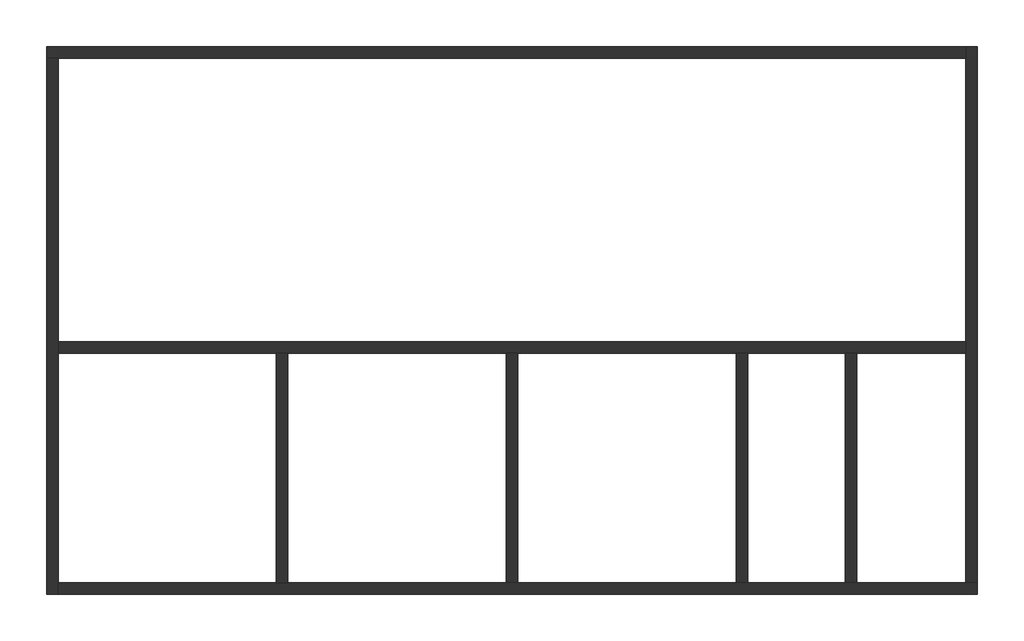
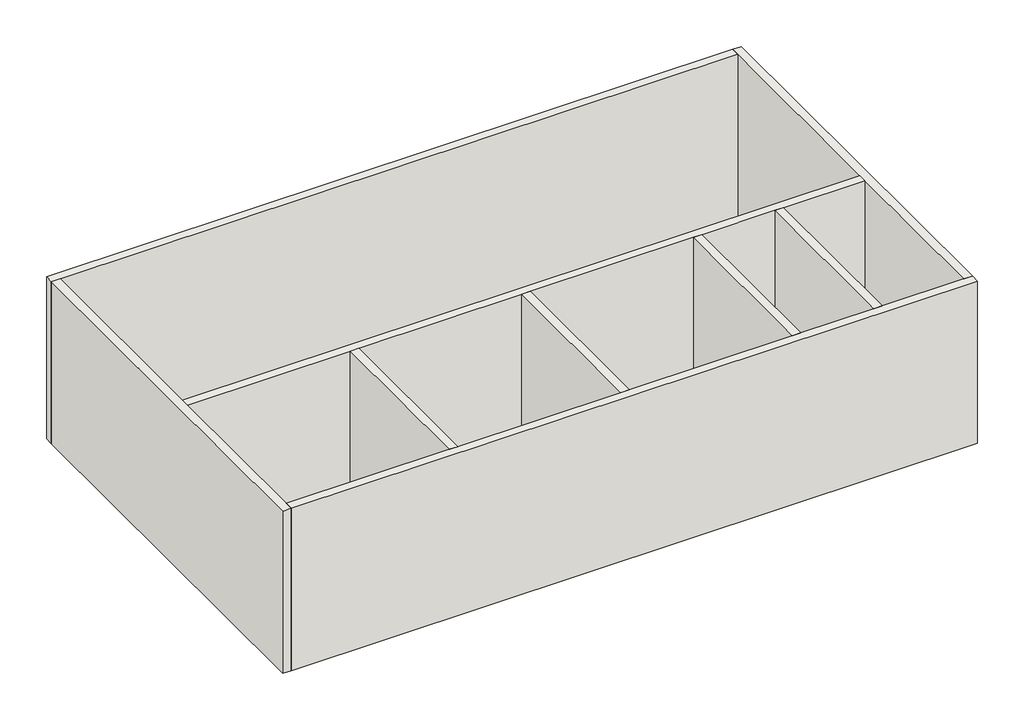
# One storey: 9 walls.
"""IFC4 building model written with IfcOpenShell, lengths in millimetres."""

from ifc_helpers import new_model, si_unit, origin, origin_with_axes, place, context, project, spatial, polyline, outline, extrude, faceted_brep, element, save

model = new_model("IFC4")

# Units and contexts
model_context = context("Model", 3, world=origin())
ifc_project = project(units=[si_unit("LENGTHUNIT", "METRE", prefix="MILLI")], contexts=[model_context])

# Site, building, storey
site = spatial("IfcSite", under=ifc_project)
building = spatial("IfcBuilding", under=site)
storey = spatial("IfcBuildingStorey", under=building, Name="1st FL GL+200", Elevation=0.0)

# Walls
placement = place(None, origin())
element("IfcWall", 1, ObjectType="일반 - 300mm", at=placement, inside=storey, context=model_context, shape_type="Brep", body=[
    faceted_brep([(-18845.7273237, 9285.9763125, 0.0), (-18545.7273237, 9285.9763125, 0.0), (5154.2726763, 9285.9763125, 0.0), (5154.2726763, 9285.9763125, 6000.0), (-18545.7273237, 9285.9763125, 6000.0), (-18845.7273237, 9285.9763125, 6000.0), (-18845.7273237, 9585.9763125, 0.0), (-18845.7273237, 9585.9763125, 6000.0), (5154.2726763, 9585.9763125, 6000.0), (5154.2726763, 9585.9763125, 0.0)], [[[0, 1, 2, 3, 4, 5]], [[6, 7, 8, 9]], [[2, 1, 0, 6, 9]], [[5, 4, 3, 8, 7]], [[0, 5, 7, 6]], [[3, 2, 9, 8]]]),
])
element("IfcWall", 2, ObjectType="일반 - 300mm", at=placement, inside=storey, context=model_context, shape_type="Brep", body=[
    faceted_brep([(-18545.7273237, -4714.0236875, 0.0), (-18545.7273237, -4414.0236875, 0.0), (-18545.7273237, 1585.9763125, 0.0), (-18545.7273237, 1885.9763125, 0.0), (-18545.7273237, 9285.9763125, 0.0), (-18545.7273237, 9285.9763125, 6000.0), (-18545.7273237, 1885.9763125, 6000.0), (-18545.7273237, 1585.9763125, 6000.0), (-18545.7273237, -4414.0236875, 6000.0), (-18545.7273237, -4714.0236875, 6000.0), (-18845.7273237, -4714.0236875, 0.0), (-18845.7273237, -4714.0236875, 6000.0), (-18845.7273237, 9285.9763125, 6000.0), (-18845.7273237, 9285.9763125, 0.0)], [[[0, 1, 2, 3, 4, 5, 6, 7, 8, 9]], [[10, 11, 12, 13]], [[4, 3, 2, 1, 0, 10, 13]], [[9, 8, 7, 6, 5, 12, 11]], [[0, 9, 11, 10]], [[5, 4, 13, 12]]]),
])
element("IfcWall", 3, ObjectType="일반 - 300mm", at=placement, inside=storey, context=model_context, shape_type="Brep", body=[
    faceted_brep([(5454.2726763, -4414.0236875, 0.0), (5154.2726763, -4414.0236875, 0.0), (2304.2726763, -4414.0236875, 0.0), (2004.2726763, -4414.0236875, 0.0), (-545.7273237, -4414.0236875, 0.0), (-845.7273237, -4414.0236875, 0.0), (-6545.7273237, -4414.0236875, 0.0), (-6845.7273237, -4414.0236875, 0.0), (-12545.7273237, -4414.0236875, 0.0), (-12845.7273237, -4414.0236875, 0.0), (-18545.7273237, -4414.0236875, 0.0), (-18545.7273237, -4414.0236875, 6000.0), (-12845.7273237, -4414.0236875, 6000.0), (-12545.7273237, -4414.0236875, 6000.0), (-6845.7273237, -4414.0236875, 6000.0), (-6545.7273237, -4414.0236875, 6000.0), (-845.7273237, -4414.0236875, 6000.0), (-545.7273237, -4414.0236875, 6000.0), (2004.2726763, -4414.0236875, 6000.0), (2304.2726763, -4414.0236875, 6000.0), (5154.2726763, -4414.0236875, 6000.0), (5454.2726763, -4414.0236875, 6000.0), (5454.2726763, -4714.0236875, 0.0), (5454.2726763, -4714.0236875, 6000.0), (-18545.7273237, -4714.0236875, 6000.0), (-18545.7273237, -4714.0236875, 0.0)], [[[0, 1, 2, 3, 4, 5, 6, 7, 8, 9, 10, 11, 12, 13, 14, 15, 16, 17, 18, 19, 20, 21]], [[22, 23, 24, 25]], [[10, 9, 8, 7, 6, 5, 4, 3, 2, 1, 0, 22, 25]], [[21, 20, 19, 18, 17, 16, 15, 14, 13, 12, 11, 24, 23]], [[0, 21, 23, 22]], [[11, 10, 25, 24]]]),
])
element("IfcWall", 4, ObjectType="일반 - 300mm", at=placement, inside=storey, context=model_context, shape_type="Brep", body=[
    faceted_brep([(5154.2726763, 9585.9763125, 0.0), (5154.2726763, 9285.9763125, 0.0), (5154.2726763, 1885.9763125, 0.0), (5154.2726763, 1585.9763125, 0.0), (5154.2726763, -4414.0236875, 0.0), (5154.2726763, -4414.0236875, 6000.0), (5154.2726763, 1585.9763125, 6000.0), (5154.2726763, 1885.9763125, 6000.0), (5154.2726763, 9285.9763125, 6000.0), (5154.2726763, 9585.9763125, 6000.0), (5454.2726763, 9585.9763125, 0.0), (5454.2726763, 9585.9763125, 6000.0), (5454.2726763, -4414.0236875, 6000.0), (5454.2726763, -4414.0236875, 0.0)], [[[0, 1, 2, 3, 4, 5, 6, 7, 8, 9]], [[10, 11, 12, 13]], [[4, 3, 2, 1, 0, 10, 13]], [[9, 8, 7, 6, 5, 12, 11]], [[0, 9, 11, 10]], [[5, 4, 13, 12]]]),
])
element("IfcWall", 5, ObjectType="일반 - 300mm", at=placement, inside=storey, context=model_context, shape_type="Brep", body=[
    faceted_brep([(-18545.7273237, 1585.9763125, 0.0), (-12845.7273237, 1585.9763125, 0.0), (-12545.7273237, 1585.9763125, 0.0), (-6845.7273237, 1585.9763125, 0.0), (-6545.7273237, 1585.9763125, 0.0), (-845.7273237, 1585.9763125, 0.0), (-545.7273237, 1585.9763125, 0.0), (2004.2726763, 1585.9763125, 0.0), (2304.2726763, 1585.9763125, 0.0), (5154.2726763, 1585.9763125, 0.0), (5154.2726763, 1585.9763125, 6000.0), (2304.2726763, 1585.9763125, 6000.0), (2004.2726763, 1585.9763125, 6000.0), (-545.7273237, 1585.9763125, 6000.0), (-845.7273237, 1585.9763125, 6000.0), (-6545.7273237, 1585.9763125, 6000.0), (-6845.7273237, 1585.9763125, 6000.0), (-12545.7273237, 1585.9763125, 6000.0), (-12845.7273237, 1585.9763125, 6000.0), (-18545.7273237, 1585.9763125, 6000.0), (-18545.7273237, 1885.9763125, 0.0), (-18545.7273237, 1885.9763125, 6000.0), (5154.2726763, 1885.9763125, 6000.0), (5154.2726763, 1885.9763125, 0.0)], [[[0, 1, 2, 3, 4, 5, 6, 7, 8, 9, 10, 11, 12, 13, 14, 15, 16, 17, 18, 19]], [[20, 21, 22, 23]], [[9, 8, 7, 6, 5, 4, 3, 2, 1, 0, 20, 23]], [[19, 18, 17, 16, 15, 14, 13, 12, 11, 10, 22, 21]], [[10, 9, 23, 22]], [[0, 19, 21, 20]]]),
])
element("IfcWall", 6, ObjectType="일반 - 300mm", at=placement, inside=storey, context=model_context, shape_type="SweptSolid", body=[
    extrude(outline(polyline([(2004.2726763, -4414.0236875), (2004.2726763, 1585.9763125), (2304.2726763, 1585.9763125), (2304.2726763, -4414.0236875), (2004.2726763, -4414.0236875)])), origin_with_axes(), (0.0, 0.0, 1.0), 6000.0),
])
element("IfcWall", 7, ObjectType="일반 - 300mm", at=placement, inside=storey, context=model_context, shape_type="SweptSolid", body=[
    extrude(outline(polyline([(-845.7273237, -4414.0236875), (-845.7273237, 1585.9763125), (-545.7273237, 1585.9763125), (-545.7273237, -4414.0236875), (-845.7273237, -4414.0236875)])), origin_with_axes(), (0.0, 0.0, 1.0), 6000.0),
])
element("IfcWall", 8, ObjectType="일반 - 300mm", at=placement, inside=storey, context=model_context, shape_type="SweptSolid", body=[
    extrude(outline(polyline([(-6845.7273237, -4414.0236875), (-6845.7273237, 1585.9763125), (-6545.7273237, 1585.9763125), (-6545.7273237, -4414.0236875), (-6845.7273237, -4414.0236875)])), origin_with_axes(), (0.0, 0.0, 1.0), 6000.0),
])
element("IfcWall", 9, ObjectType="일반 - 300mm", at=placement, inside=storey, context=model_context, shape_type="SweptSolid", body=[
    extrude(outline(polyline([(-12845.7273237, -4414.0236875), (-12845.7273237, 1585.9763125), (-12545.7273237, 1585.9763125), (-12545.7273237, -4414.0236875), (-12845.7273237, -4414.0236875)])), origin_with_axes(), (0.0, 0.0, 1.0), 6000.0),
])

save(model, "model.ifc")

# Revit data of these elements
# Project information
#   프로젝트 발행 날짜 = "발행 날짜"
#   프로젝트 상태 = "프로젝트 상태"
#   클라이언트 이름 = "소유자"
#   프로젝트 주소 = "주소를 여기에 입력"
#   프로젝트 이름 = "프로젝트 이름"
#   프로젝트 번호 = "0001"
# Grids (mm)
#   "Y16": line (2154.273, 3257.871) -> (2154.273, -8233.19)
#   "X2": line (-12695.727, -8233.19) -> (-12695.727, 14438.726)
#   "X3": line (-6695.727, -8233.19) -> (-6695.727, 14438.726)
#   "X4": line (-695.727, -8233.19) -> (-695.727, 14438.726)
#   "X5": line (5304.273, -8233.19) -> (5304.273, 14438.726)
#   "Y2": line (9794.388, 1735.976) -> (-24604.07, 1735.976)
#   "Y1": line (9794.388, -4564.024) -> (-24604.07, -4564.024)
#   "Y3": line (9794.388, 9435.976) -> (-24604.07, 9435.976)
#   "X1": line (-18695.727, -8233.19) -> (-18695.727, 14438.726)
# Type "일반 - 300mm"
#   Layers, outside or top first: 300 mm no material (function 1)
# Elements 1, 2, 3, 4, 5, 6, 7, 8, 9 (IfcWall, "일반 - 300mm")
#   Comments = ""
#   Top Offset = 0 mm
#   Base Offset = 0 mm
#   wall height = 6000 mm
#   Phase Created = 신축
#   Base Constraint = 1st FL GL+200
#   Top Constraint = 2nd FL GL+6,200
#   Materials on its faces: "기본 벽"
# Materials
#   "기본 벽": class "다양한", colour RGB 128 128 128, transparency 0, Cost = 0
# Room at (-6695.727, 5585.976) mm, phase "신축", upper level "1st FL GL+200", upper offset 6000 mm, lower offset 0 mm
#   Base Finish = "B01"
#   Ceiling Finish = "C95A"
#   Wall Finish = "W01B"
#   Floor Finish = "F03"
#   Number = "1101"
#   Name = "test"
#   Wall Base Material = "Masonry Wall"
#   Wall Finish 1 = "Plastering"
#   Wall Finish 2 = "Acrylic Emulsion Paint"
#   Wall Finish Remark = "THK 12 Plaster"
#   Floor Base Material = "Concrete Slab"
#   Floor Finish 1 = "Steel Trowel Finish"
#   Floor Finish 2 = "Acid Resistant Paint"
#   Base Base Material = "Concrete Wall"
#   Base Finish 1 = "Acrylic Emulsion Paint"
#   Base Finish Remark = "H=100"
#   Ceiling Base Material = "Concrete Slab"
#   Ceiling Finish 1 = "Acoustic Tiled Ceiling System (T-Bar)"
#   Ceiling Finish Remark = "600x600, CH=3000"
#   H_Room W = 0 mm
#   H_Room L = 0 mm
#   H_Room H or CH = 0 mm
#   Wall Finish Style = Acrylic Emulsion Paint on Cement Plaster
#   Floor Finish Style = Acid Resistant Paint on Steel Trowel Finish
#   Base Finish Style = Acrylic Emulsion Paint
#   Ceiling Finish Style = Suspended Acoustic Tiled Ceiling (T-Bar)
# Room at (3729.273, -1414.024) mm, phase "신축", upper level "1st FL GL+200", upper offset 6000 mm, lower offset 0 mm
#   Base Finish = "B03"
#   Ceiling Finish = "C95A"
#   Wall Finish = "W01B"
#   Floor Finish = "F06A"
#   Number = "1102"
#   Name = "test"
#   H_Room W = 0 mm
#   H_Room L = 0 mm
#   H_Room H or CH = 0 mm
# Room at (729.273, -1414.024) mm, phase "신축", upper level "1st FL GL+200", upper offset 6000 mm, lower offset 0 mm
#   Base Finish = "B32"
#   Ceiling Finish = "C96A"
#   Wall Finish = "W04B"
#   Floor Finish = "F31B"
#   Number = "1103"
#   Name = "test"
#   H_Room W = 0 mm
#   H_Room L = 0 mm
#   H_Room H or CH = 0 mm
# Room at (-3695.727, -1414.024) mm, phase "신축", upper level "1st FL GL+200", upper offset 6000 mm, lower offset 0 mm
#   Base Finish = "B33"
#   Ceiling Finish = "C01"
#   Wall Finish = "W32D"
#   Floor Finish = "F34A"
#   Number = "1104"
#   Name = "test"
#   H_Room W = 0 mm
#   H_Room L = 0 mm
#   H_Room H or CH = 0 mm
# Room at (-15695.727, -1414.024) mm, phase "신축", upper level "1st FL GL+200", upper offset 6000 mm, lower offset 0 mm
#   Base Finish = "B01"
#   Ceiling Finish = "C96A"
#   Wall Finish = "W01B"
#   Floor Finish = "F41"
#   Number = "1106"
#   Name = "test"
#   H_Room W = 0 mm
#   H_Room L = 0 mm
#   H_Room H or CH = 0 mm
# Room at (-9695.727, -1414.024) mm, phase "신축", upper level "1st FL GL+200", upper offset 6000 mm, lower offset 0 mm
#   Base Finish = "B35A"
#   Ceiling Finish = "C95A"
#   Wall Finish = "W01A"
#   Floor Finish = "F34B"
#   Number = "1105"
#   Name = "test"
#   H_Room W = 0 mm
#   H_Room L = 0 mm
#   H_Room H or CH = 0 mm
